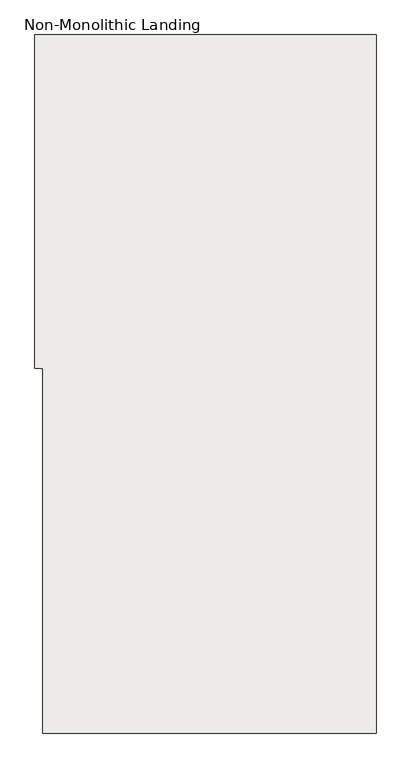
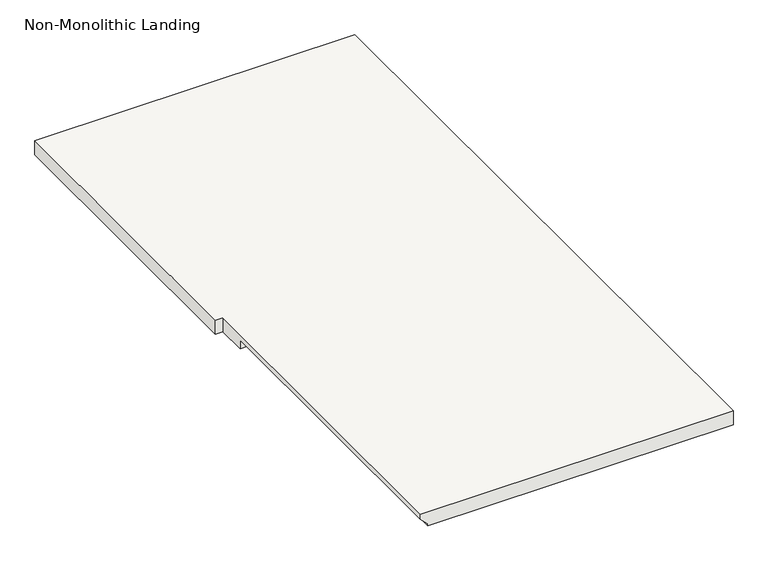
"""IFC4 building model written with IfcOpenShell, lengths in millimetres: slab geometry, Non-Monolithic Landing."""

from ifc_helpers import new_model, si_unit, origin, place, context, project, spatial, faceted_brep, source, transform, mapped, element, save


def non_monolithic_landing_31b71f01(model_context):
    return source(origin(), model_context, "Body", "Brep", [
        faceted_brep([(665981.788677, -551651.2413841, 1549.5716216), (665956.388677, -551651.2413841, 1574.9716216), (665956.388677, -550584.4413841, 1574.9716216), (665981.788677, -550584.4413841, 1549.5716216), (667023.188677, -551651.2413841, 1594.0216216), (667023.188677, -549416.0413841, 1594.0216216), (665956.388677, -549416.0413841, 1594.0216216), (665930.988677, -549416.0413841, 1594.0216216), (665930.988677, -550482.8413841, 1594.0216216), (665956.388677, -550482.8413841, 1594.0216216), (665956.388677, -551651.2413841, 1594.0216216), (665981.788677, -550584.4413841, 1543.2216216), (665956.388677, -550584.4413841, 1543.2216216), (665956.388677, -550482.8413841, 1543.2216216), (665930.988677, -550482.8413841, 1543.2216216), (665930.988677, -549416.0413841, 1543.2216216), (665956.388677, -549416.0413841, 1543.2216216), (667023.188677, -549416.0413841, 1543.2216216), (667023.188677, -551651.2413841, 1543.2216216), (665981.788677, -551651.2413841, 1543.2216216)], [[[0, 1, 2, 3]], [[4, 5, 6, 7, 8, 9, 10]], [[11, 12, 13, 14, 15, 16, 17, 18, 19]], [[12, 11, 3, 2]], [[11, 19, 0, 3]], [[4, 10, 1, 0, 19, 18]], [[5, 4, 18, 17]], [[6, 5, 17, 16]], [[7, 6, 16, 15]], [[8, 7, 15, 14]], [[9, 8, 14, 13]], [[10, 9, 13, 12, 2, 1]]]),
    ])


if __name__ == "__main__":
    model = new_model("IFC4")
    model_context = context("Model", 3, world=origin())
    ifc_project = project(units=[si_unit("LENGTHUNIT", "METRE", prefix="MILLI")], contexts=[model_context])
    site = spatial("IfcSite", under=ifc_project)
    building = spatial("IfcBuilding", under=site)
    placement = place(None, origin())
    non_monolithic_landing_shape = non_monolithic_landing_31b71f01(model_context)
    element("IfcSlab", 1, ObjectType="Non-Monolithic Landing", at=placement, inside=building, context=model_context, shape_type="MappedRepresentation", body=[
        mapped(non_monolithic_landing_shape, transform((0.0, 0.0, 0.0), x_axis=(1.0, 0.0, 0.0), y_axis=(0.0, 1.0, 0.0), z_axis=(0.0, 0.0, 1.0))),
    ])
    save(model, "model.ifc")
